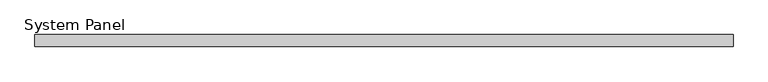
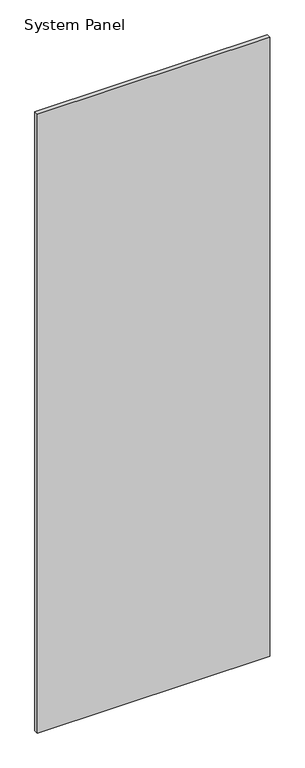
"""IFC4 building model written with IfcOpenShell, lengths in millimetres: plate geometry, System Panel : WWm-Glass-20mm-10mmOffset."""

from ifc_helpers import new_model, si_unit, origin, origin_with_axes, place, context, project, spatial, polyline, outline, extrude, source, transform, mapped, element, save


def system_panel_c1c6b796(model_context):
    return source(origin(), model_context, "Body", "SweptSolid", [
        extrude(outline(polyline([(577.5, 0.0), (-577.5, 0.0), (-577.5, 20.0), (577.5, 20.0), (577.5, 0.0)])), origin_with_axes(), (0.0, 0.0, 1.0), 3250.0),
    ])


if __name__ == "__main__":
    model = new_model("IFC4")
    model_context = context("Model", 3, world=origin())
    ifc_project = project(units=[si_unit("LENGTHUNIT", "METRE", prefix="MILLI")], contexts=[model_context])
    site = spatial("IfcSite", under=ifc_project)
    building = spatial("IfcBuilding", under=site)
    placement = place(None, origin())
    system_panel_shape = system_panel_c1c6b796(model_context)
    element("IfcPlate", 1, ObjectType="System Panel : WWm-Glass-20mm-10mmOffset", at=placement, inside=building, context=model_context, shape_type="MappedRepresentation", body=[
        mapped(system_panel_shape, transform((0.0, 0.0, 0.0), x_axis=(1.0, 0.0, 0.0), y_axis=(0.0, 1.0, 0.0), z_axis=(0.0, 0.0, 1.0))),
    ])
    save(model, "model.ifc")

# Revit data of these elements
# Type "System Panel : WWm-Glass-20mm-10mmOffset"
#   Finish = ""
# Element 1 (IfcPlate, "System Panel : WWm-Glass-20mm-10mmOffset")
#   Materials on its faces: "WW-EC-GL-Storefront"
# Materials
#   "WW-EC-GL-Storefront": class "Glass", colour RGB 236 240 239, transparency 0.85, Description = "Storefront Glass", Cost = 0
